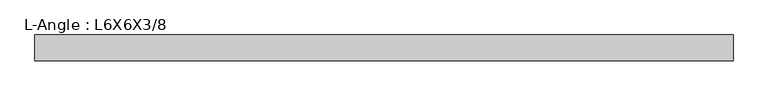
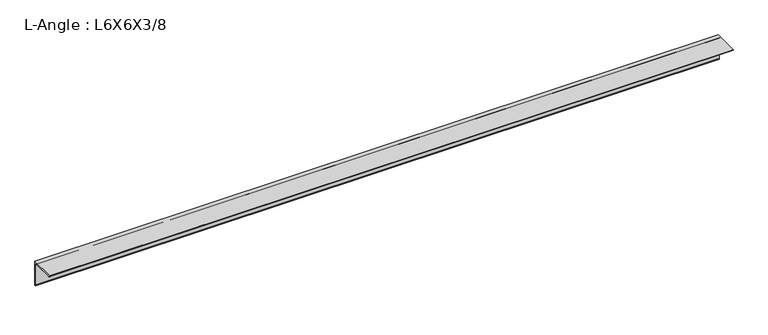
"""IFC4 building model written with IfcOpenShell, lengths in millimetres: member geometry, L-Angle : L6X6X3/8."""

import ifcopenshell
import ifcopenshell.guid

model = None  # the IFC model being written
_history = None  # IfcOwnerHistory: only IFC2X3 demands one
_inside = {}  # id of a spatial element -> (the spatial element, [elements in it])
_under = {}  # id of a project, library or spatial element -> (it, [spatial elements below it])
_declared = {}  # id of a project -> (the project, [libraries it declares])
_typed = {}  # id of a type object -> (the type object, [elements of that type])
_made_of = {}  # id of a material, layer set ... -> (it, [elements and type objects made of it])


def new_model(schema):
    """Start an empty IFC model of exactly this schema.

    Asked for "IFC4X3", IfcOpenShell would pick the latest addendum, in which some entities
    have other attributes; the version numbers below select the first issue.
    IFC2X3 requires an IfcOwnerHistory on every rooted entity: one is made here for all.
    """
    global model, _history
    if schema == "IFC4X3":
        model = ifcopenshell.file(schema_version=(4, 3, 0, 0))
    else:
        model = ifcopenshell.file(schema=schema)
    _inside.clear()
    _under.clear()
    _declared.clear()
    _typed.clear()
    _made_of.clear()
    _history = None
    if model.schema == "IFC2X3":
        org = make("IfcOrganization", Name="unknown")
        user = make(
            "IfcPersonAndOrganization",
            ThePerson=make("IfcPerson", FamilyName="unknown"),
            TheOrganization=org,
        )
        app = make(
            "IfcApplication",
            ApplicationDeveloper=org,
            Version="unknown",
            ApplicationFullName="unknown",
            ApplicationIdentifier="unknown",
        )
        _history = make(
            "IfcOwnerHistory",
            OwningUser=user,
            OwningApplication=app,
            ChangeAction="ADDED",
            CreationDate=0,
        )
    return model


def make(cls, **values):
    """One entity of the class cls with the attributes given. An attribute that is None is left unset."""
    return model.create_entity(
        cls, **{name: value for name, value in values.items() if value is not None}
    )


def rooted(cls, **values):
    """An entity with a GlobalId (a new one), such as an element, a storey or a relation."""
    return make(cls, GlobalId=ifcopenshell.guid.new(), OwnerHistory=_history, **values)


def si_unit(unit_type, name, prefix=None):
    """IfcSIUnit, for example si_unit("LENGTHUNIT", "METRE", prefix="MILLI")."""
    return make("IfcSIUnit", UnitType=unit_type, Prefix=prefix, Name=name)


def assignment(units):
    """IfcUnitAssignment: the units of a project."""
    return None if units is None else make("IfcUnitAssignment", Units=units)


def point(xyz):
    """IfcCartesianPoint."""
    return None if xyz is None else make("IfcCartesianPoint", Coordinates=xyz)


def direction(xyz):
    """IfcDirection."""
    return None if xyz is None else make("IfcDirection", DirectionRatios=xyz)


def frame(location, z_axis=None, x_axis=None):
    """IfcAxis2Placement3D, a coordinate frame: its origin and axes. An axis left out is left unset."""
    return make(
        "IfcAxis2Placement3D",
        Location=point(location),
        Axis=direction(z_axis),
        RefDirection=direction(x_axis),
    )


def frame_2d(location, x_axis=None):
    """IfcAxis2Placement2D, a coordinate frame in the plane: its origin and x axis."""
    return make(
        "IfcAxis2Placement2D", Location=point(location), RefDirection=direction(x_axis)
    )


def origin():
    """The frame at (0, 0, 0) with its axes left unset."""
    return frame((0.0, 0.0, 0.0))


def place(relative_to, where):
    """IfcLocalPlacement: puts the frame where relative to a parent placement (None: the world)."""
    return make(
        "IfcLocalPlacement", PlacementRelTo=relative_to, RelativePlacement=where
    )


def context(
    kind, dimensions, precision=None, world=None, true_north=None, identifier=None
):
    """IfcGeometricRepresentationContext, for example the 3D "Model" context."""
    return make(
        "IfcGeometricRepresentationContext",
        ContextIdentifier=identifier,
        ContextType=kind,
        CoordinateSpaceDimension=dimensions,
        Precision=precision,
        WorldCoordinateSystem=world,
        TrueNorth=true_north,
    )


def project(units=None, contexts=None):
    """IfcProject with its units and contexts."""
    return rooted(
        "IfcProject",
        Name="project",
        RepresentationContexts=contexts,
        UnitsInContext=assignment(units),
    )


def spatial(cls, under=None, at=None, **own):
    """A site, building, storey or space (cls), placed at a placement, below another one or the project."""
    s = rooted(cls, ObjectPlacement=at, **own)
    if under is not None:
        _under.setdefault(under.id(), (under, []))[1].append(s)
    return s


def polyline(points):
    """IfcPolyline through the points."""
    return make("IfcPolyline", Points=[point(p) for p in points])


def circle_curve(where, radius):
    """IfcCircle in the frame where."""
    return make("IfcCircle", Position=where, Radius=radius)


def trimmed(basis, trim1, trim2, sense, master):
    """IfcTrimmedCurve: the piece of a basis curve between two trims."""
    return make(
        "IfcTrimmedCurve",
        BasisCurve=basis,
        Trim1=trim1,
        Trim2=trim2,
        SenseAgreement=sense,
        MasterRepresentation=master,
    )


def segment(curve, same_sense, transition):
    """IfcCompositeCurveSegment."""
    return make(
        "IfcCompositeCurveSegment",
        Transition=transition,
        SameSense=same_sense,
        ParentCurve=curve,
    )


def composite_curve(segments, self_intersect=None):
    """IfcCompositeCurve: segments joined end to end."""
    return make("IfcCompositeCurve", Segments=segments, SelfIntersect=self_intersect)


def outline(outer, holes=None, kind="AREA"):
    """IfcArbitraryClosedProfileDef: a profile drawn as a closed curve; with holes, ...WithVoids."""
    if holes is None:
        return make("IfcArbitraryClosedProfileDef", ProfileType=kind, OuterCurve=outer)
    return make(
        "IfcArbitraryProfileDefWithVoids",
        ProfileType=kind,
        OuterCurve=outer,
        InnerCurves=holes,
    )


def extrude(swept, where, along, depth):
    """IfcExtrudedAreaSolid: the profile swept, set in the frame where, extruded along a direction by depth."""
    return make(
        "IfcExtrudedAreaSolid",
        SweptArea=swept,
        Position=where,
        ExtrudedDirection=direction(along),
        Depth=depth,
    )


def shape(context_of_items, identifier, shape_type, items):
    """IfcShapeRepresentation: the items that make up one representation, for example the "Body"."""
    return make(
        "IfcShapeRepresentation",
        ContextOfItems=context_of_items,
        RepresentationIdentifier=identifier,
        RepresentationType=shape_type,
        Items=items,
    )


def source(mapping_origin, context_of_items, identifier, shape_type, items):
    """IfcRepresentationMap: a shape defined once, which mapped items show again and again."""
    return make(
        "IfcRepresentationMap",
        MappingOrigin=mapping_origin,
        MappedRepresentation=shape(context_of_items, identifier, shape_type, items),
    )


def transform(
    local_origin,
    x_axis=None,
    y_axis=None,
    z_axis=None,
    scale=None,
    scale2=None,
    scale3=None,
    uniform=True,
):
    """IfcCartesianTransformationOperator3D, or its non-uniform kind. x_axis, y_axis, z_axis: its Axis1, 2, 3."""
    if uniform:
        return make(
            "IfcCartesianTransformationOperator3D",
            Axis1=direction(x_axis),
            Axis2=direction(y_axis),
            LocalOrigin=point(local_origin),
            Scale=scale,
            Axis3=direction(z_axis),
        )
    return make(
        "IfcCartesianTransformationOperator3DnonUniform",
        Axis1=direction(x_axis),
        Axis2=direction(y_axis),
        LocalOrigin=point(local_origin),
        Scale=scale,
        Axis3=direction(z_axis),
        Scale2=scale2,
        Scale3=scale3,
    )


def mapped(mapping_source, mapping_target):
    """IfcMappedItem: shows the shape of a source again, moved by a transform."""
    return make(
        "IfcMappedItem", MappingSource=mapping_source, MappingTarget=mapping_target
    )


def made_of(thing, what):
    """Note that an element or type object is made of a material, layer set ...; save() writes the relation."""
    if what is not None:
        _made_of.setdefault(what.id(), (what, []))[1].append(thing)
    return thing


def element(
    cls,
    number,
    at=None,
    inside=None,
    cuts=None,
    type_object=None,
    material=None,
    context=None,
    identifier="Body",
    shape_type=None,
    held_by="IfcProductDefinitionShape",
    body=None,
    shapes=None,
    **own,
):
    """One element of the class cls, such as IfcWall. Its Tag is "e" and its number.

    at: its placement. inside: the storey or other place that contains it. cuts: it is an
    opening in that element (IfcRelVoidsElement). A single representation is given by context,
    identifier, shape_type and body (its items); several are given by shapes. held_by: the class
    of the entity that holds the representations. save() writes the other relations.
    """
    e = rooted(cls, Tag="e%d" % number, ObjectPlacement=at, **own)
    if body is not None:
        shapes = [shape(context, identifier, shape_type, body)]
    if shapes is not None:
        e.Representation = make(held_by, Representations=shapes)
    if inside is not None:
        _inside.setdefault(inside.id(), (inside, []))[1].append(e)
    if cuts is not None:
        rooted(
            "IfcRelVoidsElement", RelatingBuildingElement=cuts, RelatedOpeningElement=e
        )
    if type_object is not None:
        _typed.setdefault(type_object.id(), (type_object, []))[1].append(e)
    return made_of(e, material)


def aggregate(whole, parts):
    """IfcRelAggregates: a whole, such as a stair, and the parts it consists of."""
    return rooted("IfcRelAggregates", RelatingObject=whole, RelatedObjects=parts)


def save(model, path):
    """Write the relations noted so far, then the file.

    IfcRelAggregates (storeys below a building ...), IfcRelContainedInSpatialStructure (elements
    in a storey), IfcRelDefinesByType, IfcRelAssociatesMaterial and IfcRelDeclares: one each for
    every whole, place, type object, material and project.
    """
    for whole, parts in _under.values():
        aggregate(whole, parts)
    for where, things in _inside.values():
        rooted(
            "IfcRelContainedInSpatialStructure",
            RelatedElements=things,
            RelatingStructure=where,
        )
    for kind, things in _typed.values():
        rooted("IfcRelDefinesByType", RelatedObjects=things, RelatingType=kind)
    for what, things in _made_of.values():
        rooted("IfcRelAssociatesMaterial", RelatedObjects=things, RelatingMaterial=what)
    for by, libraries in _declared.values():
        rooted("IfcRelDeclares", RelatingContext=by, RelatedDefinitions=libraries)
    model.write(path)


def l_angle_l6x6x3_8_1e5b70da(model_context):
    return source(origin(), model_context, "Body", "SweptSolid", [
        extrude(outline(composite_curve([segment(polyline([(41.148, 41.148), (41.148, -111.252)]), True, "CONTINUOUS"), segment(trimmed(circle_curve(frame_2d((41.148, -101.727)), 9.525), [point((41.148, -111.252))], [point((31.623, -101.727))], False, "CARTESIAN"), True, "CONTINUOUS"), segment(polyline([(31.623, -101.727), (31.623, 22.098)]), True, "CONTINUOUS"), segment(trimmed(circle_curve(frame_2d((22.098, 22.098)), 9.525), [point((31.623, 22.098))], [point((22.098, 31.623))], True, "CARTESIAN"), True, "CONTINUOUS"), segment(polyline([(22.098, 31.623), (-101.727, 31.623)]), True, "CONTINUOUS"), segment(trimmed(circle_curve(frame_2d((-101.727, 41.148)), 9.525), [point((-101.727, 31.623))], [point((-111.252, 41.148))], False, "CARTESIAN"), True, "CONTINUOUS"), segment(polyline([(-111.252, 41.148), (41.148, 41.148)]), True, "CONTINUOUS")], self_intersect=False)), frame((-2053.4214347, 0.0, 0.0), z_axis=(1.0, 0.0, 0.0), x_axis=(0.0, 1.0, 0.0)), (0.0, 0.0, 1.0), 4092.1699392),
    ])


if __name__ == "__main__":
    model = new_model("IFC4")
    model_context = context("Model", 3, world=origin())
    ifc_project = project(units=[si_unit("LENGTHUNIT", "METRE", prefix="MILLI")], contexts=[model_context])
    site = spatial("IfcSite", under=ifc_project)
    building = spatial("IfcBuilding", under=site)
    placement = place(None, origin())
    l_angle_l6x6x3_8_shape = l_angle_l6x6x3_8_1e5b70da(model_context)
    element("IfcMember", 1, ObjectType="L-Angle : L6X6X3/8", at=placement, inside=building, context=model_context, shape_type="MappedRepresentation", body=[
        mapped(l_angle_l6x6x3_8_shape, transform((0.0, 0.0, 0.0), x_axis=(1.0, 0.0, 0.0), y_axis=(0.0, 1.0, 0.0), z_axis=(0.0, 0.0, 1.0))),
    ])
    save(model, "model.ifc")

# Revit data of these elements
# Type "L-Angle : L6X6X3/8"
#   Assembly Code = "B10"
#   k = 0' - 0 7/8"
#   W = 14.9
#   Length [instance default] = 5' - 0"
#   b = 0' - 6"
#   d = 0' - 6"
#   t = 0' - 0 3/8"
#   x = 0' - 1.62"
#   y = 0' - 1.62"
#   A = 0.0304167 SF
#   Structural Material [instance default] = Steel ASTM A36
# Element 1 (IfcMember, "L-Angle : L6X6X3/8")
#   Materials on its faces: "Steel ASTM A36"
# Materials
#   "Steel ASTM A36": class "Metal", colour RGB 199 199 199, transparency 0, Description = "Structural steel, ASTM A36 Grade B, mill finish", Cost = 0
